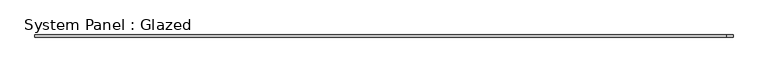
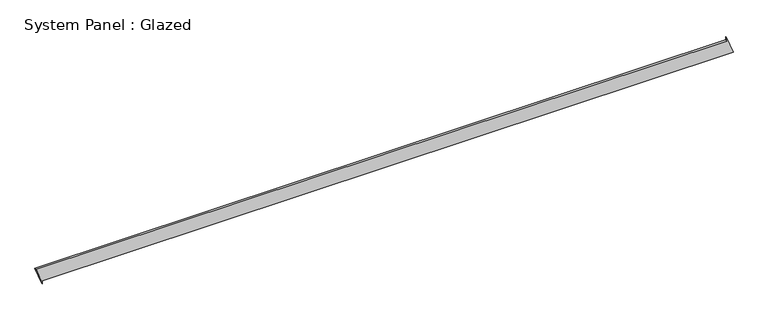
"""IFC4 building model written with IfcOpenShell, lengths in millimetres: plate geometry, System Panel : Glazed."""

from ifc_helpers import new_model, si_unit, frame, origin, place, context, project, spatial, polyline, outline, extrude, source, transform, mapped, element, save


def system_panel_glazed_43a92db8(model_context):
    return source(origin(), model_context, "Body", "SweptSolid", [
        extrude(outline(polyline([(0.0, -3956.7216602), (35.3553391, -3956.7216602), (35.3553391, 4027.3319665), (234.8589574, 3956.5179694), (199.5036184, 3956.5175852), (199.5903648, -4027.3319665), (0.0, -3956.7216602)])), frame((0.0, -49.5, 0.0), z_axis=(0.0, 1.0, 0.0), x_axis=(0.0, 0.0, 1.0)), (0.0, 0.0, 1.0), 25.0),
    ])


if __name__ == "__main__":
    model = new_model("IFC4")
    model_context = context("Model", 3, world=origin())
    ifc_project = project(units=[si_unit("LENGTHUNIT", "METRE", prefix="MILLI")], contexts=[model_context])
    site = spatial("IfcSite", under=ifc_project)
    building = spatial("IfcBuilding", under=site)
    placement = place(None, origin())
    system_panel_glazed_shape = system_panel_glazed_43a92db8(model_context)
    element("IfcPlate", 1, ObjectType="System Panel : Glazed", at=placement, inside=building, context=model_context, shape_type="MappedRepresentation", body=[
        mapped(system_panel_glazed_shape, transform((0.0, 0.0, 0.0), x_axis=(1.0, 0.0, 0.0), y_axis=(0.0, 1.0, 0.0), z_axis=(0.0, 0.0, 1.0))),
    ])
    save(model, "model.ifc")

# Revit data of these elements
# Element 1 (IfcPlate, "System Panel : Glazed")
#   Materials on its faces: "Glass"
# Materials
#   "Glass": class "Glass", colour RGB 218 227 224, transparency 0.85, Description = "Soda Lime Glass", Cost = 0
